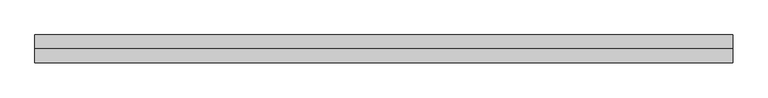
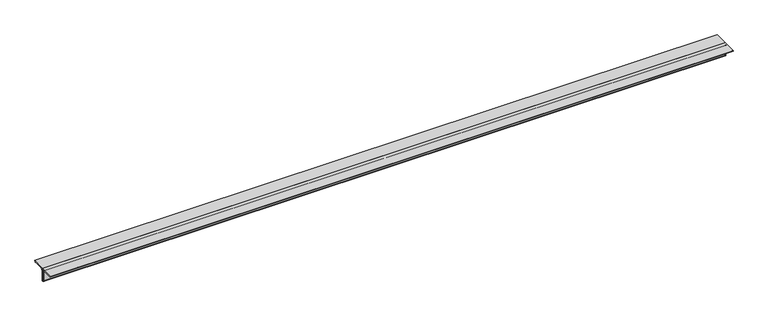
"""IFC4 building model written with IfcOpenShell, lengths in millimetres: member geometry, Steel Framing_2Ls_KS : H_SB_AR_S02_2Ls-100x100x10_VBR1."""

from ifc_helpers import new_model, si_unit, point, frame, frame_2d, origin, place, context, project, spatial, polyline, circle_curve, trimmed, segment, composite_curve, outline, extrude, source, transform, mapped, element, save


def member_f5bf67ae(model_context):
    return source(origin(), model_context, "Body", "SweptSolid", [
        extrude(outline(composite_curve([segment(polyline([(0.0, 28.2), (0.0, -71.8)]), True, "CONTINUOUS"), segment(trimmed(circle_curve(frame_2d((0.0, -61.8)), 10.0), [point((0.0, -71.8))], [point((-10.0, -61.8))], False, "CARTESIAN"), True, "CONTINUOUS"), segment(polyline([(-10.0, -61.8), (-10.0, 8.2)]), True, "CONTINUOUS"), segment(trimmed(circle_curve(frame_2d((-20.0, 8.2)), 10.0), [point((-10.0, 8.2))], [point((-20.0, 18.2))], True, "CARTESIAN"), True, "CONTINUOUS"), segment(polyline([(-20.0, 18.2), (-90.0, 18.2)]), True, "CONTINUOUS"), segment(trimmed(circle_curve(frame_2d((-90.0, 28.2)), 10.0), [point((-90.0, 18.2))], [point((-100.0, 28.2))], False, "CARTESIAN"), True, "CONTINUOUS"), segment(polyline([(-100.0, 28.2), (0.0, 28.2)]), True, "CONTINUOUS")], self_intersect=False)), frame((-2498.2204145, 0.0, 0.0), z_axis=(1.0, 0.0, 0.0), x_axis=(0.0, 1.0, 0.0)), (0.0, 0.0, 1.0), 4996.4408289),
        extrude(outline(composite_curve([segment(polyline([(0.0, 28.2), (100.0, 28.2)]), True, "CONTINUOUS"), segment(trimmed(circle_curve(frame_2d((90.0, 28.2)), 10.0), [point((100.0, 28.2))], [point((90.0, 18.2))], False, "CARTESIAN"), True, "CONTINUOUS"), segment(polyline([(90.0, 18.2), (20.0, 18.2)]), True, "CONTINUOUS"), segment(trimmed(circle_curve(frame_2d((20.0, 8.2)), 10.0), [point((20.0, 18.2))], [point((10.0, 8.2))], True, "CARTESIAN"), True, "CONTINUOUS"), segment(polyline([(10.0, 8.2), (10.0, -61.8)]), True, "CONTINUOUS"), segment(trimmed(circle_curve(frame_2d((0.0, -61.8)), 10.0), [point((10.0, -61.8))], [point((0.0, -71.8))], False, "CARTESIAN"), True, "CONTINUOUS"), segment(polyline([(0.0, -71.8), (0.0, 28.2)]), True, "CONTINUOUS")], self_intersect=False)), frame((-2498.2204145, 0.0, 0.0), z_axis=(1.0, 0.0, 0.0), x_axis=(0.0, 1.0, 0.0)), (0.0, 0.0, 1.0), 4996.4408289),
    ])


if __name__ == "__main__":
    model = new_model("IFC4")
    model_context = context("Model", 3, world=origin())
    ifc_project = project(units=[si_unit("LENGTHUNIT", "METRE", prefix="MILLI")], contexts=[model_context])
    site = spatial("IfcSite", under=ifc_project)
    building = spatial("IfcBuilding", under=site)
    placement = place(None, origin())
    member_shape = member_f5bf67ae(model_context)
    element("IfcMember", 1, ObjectType="Steel Framing_2Ls_KS : H_SB_AR_S02_2Ls-100x100x10_VBR1", at=placement, inside=building, context=model_context, shape_type="MappedRepresentation", body=[
        mapped(member_shape, transform((0.0, 0.0, 0.0), x_axis=(1.0, 0.0, 0.0), y_axis=(0.0, 1.0, 0.0), z_axis=(0.0, 0.0, 1.0))),
    ])
    save(model, "model.ifc")

# Revit data of these elements
# Type "Steel Framing_2Ls_KS : H_SB_AR_S02_2Ls-100x100x10_VBR1"
#   Type Comments = "MAIN"
#   Type Mark = "VBR1"
#   H_SectionID = "2Ls-100x100x10"
#   Assembly Code = "B10"
#   Legs = "LLBB"
#   H_Ratio for Additional Steel Plate = 0.2
#   W = 0
#   Perimeter = 0.80 m²/m
#   Nominal Weight = 29.80 kgf/m
#   Length [instance default] = 1524 mm
#   Space = 0 mm
#   b = 100 mm
#   d = 100 mm
#   t = 10 mm
#   y = 28.2 mm
#   A = 0.0038 m²
#   Structural Material [instance default] = Steel, 45-345
# Element 1 (IfcMember, "Steel Framing_2Ls_KS : H_SB_AR_S02_2Ls-100x100x10_VBR1")
#   Materials on its faces: "Steel, 45-345"
# Materials
#   "Steel, 45-345": class "Metal", colour RGB 189 187 185, transparency 0, Description = "Steel 345 MPa", Cost = 0
